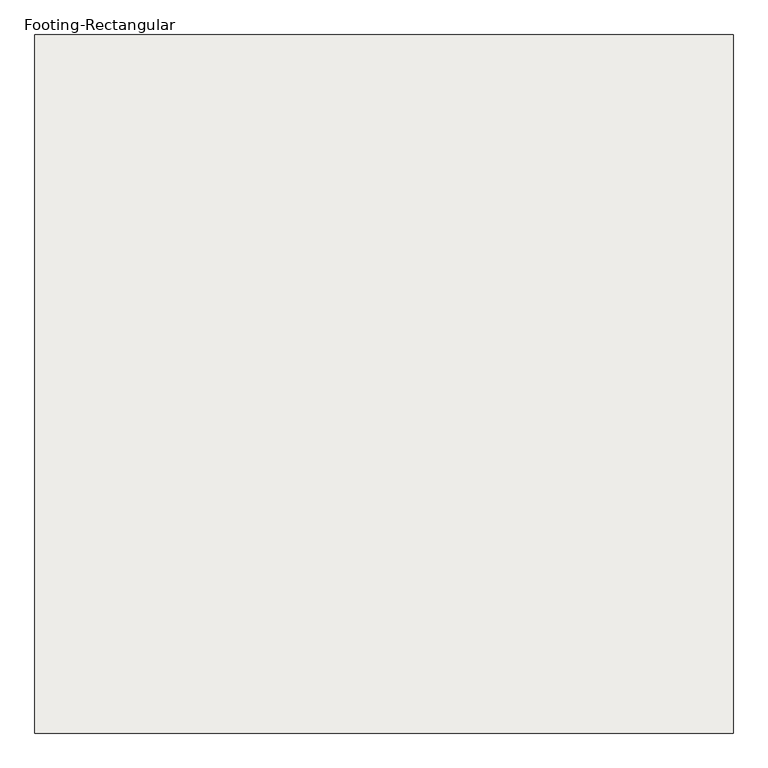
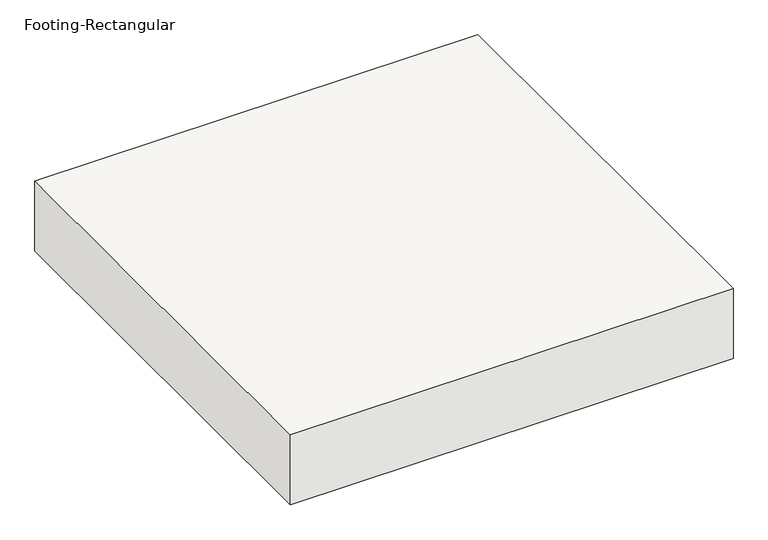
"""IFC4 building model written with IfcOpenShell, lengths in millimetres: slab geometry, Footing-Rectangular."""

from ifc_helpers import new_model, si_unit, frame, origin, place, context, project, spatial, polyline, outline, extrude, source, transform, mapped, element, save


def footing_rectangular_a4ec12e7(model_context):
    return source(origin(), model_context, "Body", "SweptSolid", [
        extrude(outline(polyline([(1828.8, 1828.8), (1828.8, -1828.8), (-1828.8, -1828.8), (-1828.8, 1828.8), (1828.8, 1828.8)])), frame((0.0, 0.0, -609.6), z_axis=(0.0, 0.0, 1.0), x_axis=(1.0, 0.0, 0.0)), (0.0, 0.0, 1.0), 609.6),
    ])


if __name__ == "__main__":
    model = new_model("IFC4")
    model_context = context("Model", 3, world=origin())
    ifc_project = project(units=[si_unit("LENGTHUNIT", "METRE", prefix="MILLI")], contexts=[model_context])
    site = spatial("IfcSite", under=ifc_project)
    building = spatial("IfcBuilding", under=site)
    placement = place(None, origin())
    footing_rectangular_shape = footing_rectangular_a4ec12e7(model_context)
    element("IfcSlab", 1, ObjectType="Footing-Rectangular : E 12' x 12' x 24\"", at=placement, inside=building, context=model_context, shape_type="MappedRepresentation", body=[
        mapped(footing_rectangular_shape, transform((0.0, 0.0, 0.0), x_axis=(1.0, 0.0, 0.0), y_axis=(0.0, 1.0, 0.0), z_axis=(0.0, 0.0, 1.0))),
    ])
    save(model, "model.ifc")

# Revit data of these elements
# Type "Footing-Rectangular : E 12' x 12' x 24\""
#   Assembly Code = "A1010100"
#   Width = 12' - 0"
#   Length = 12' - 0"
#   Foundation Thickness = 2' - 0"
#   Structural Material [instance default] = Concrete, Cast-in-Place gray
# Element 1 (IfcSlab, "Footing-Rectangular : E 12' x 12' x 24\"")
#   Materials on its faces: "Concrete, Cast-in-Place gray"
# Materials
#   "Concrete, Cast-in-Place gray": class "Concrete", colour RGB 192 192 192, transparency 0, Description = "Cast-in-place concrete", Cost = 0
